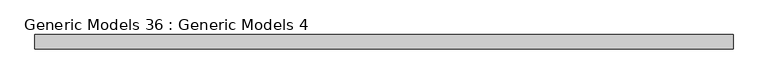
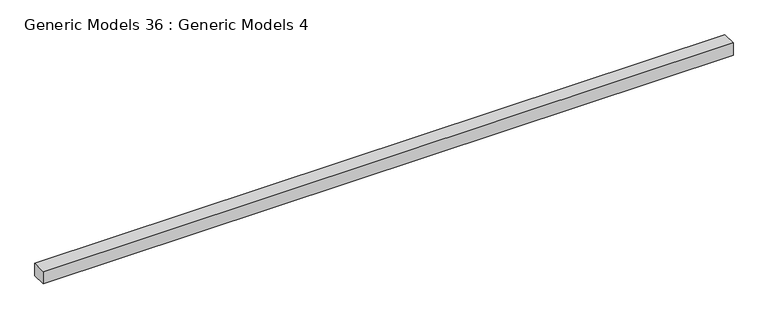
"""IFC4 building model written with IfcOpenShell, lengths in millimetres: proxy geometry, Generic Models 36 : Generic Models 4."""

from ifc_helpers import new_model, si_unit, frame, origin, place, context, project, spatial, polyline, outline, extrude, source, transform, mapped, element, save


def generic_models_36_generic_models_4_c2a80e1e(model_context):
    return source(origin(), model_context, "Body", "SweptSolid", [
        extrude(outline(polyline([(8409.0828684, 11880.2769662), (8409.0828684, 11499.2769662), (-10234.5171316, 11499.2769662), (-10234.5171316, 11880.2769662), (8409.0828684, 11880.2769662)])), frame((0.0, 0.0, 126402.846), z_axis=(0.0, 0.0, 1.0), x_axis=(1.0, 0.0, 0.0)), (0.0, 0.0, 1.0), 347.5929632),
    ])


if __name__ == "__main__":
    model = new_model("IFC4")
    model_context = context("Model", 3, world=origin())
    ifc_project = project(units=[si_unit("LENGTHUNIT", "METRE", prefix="MILLI")], contexts=[model_context])
    site = spatial("IfcSite", under=ifc_project)
    building = spatial("IfcBuilding", under=site)
    placement = place(None, origin())
    generic_models_36_generic_models_4_shape = generic_models_36_generic_models_4_c2a80e1e(model_context)
    element("IfcBuildingElementProxy", 1, Name="Generic Models 36 : Generic Models 4", ObjectType="Generic Models 36 : Generic Models 4", at=placement, inside=building, context=model_context, shape_type="MappedRepresentation", body=[
        mapped(generic_models_36_generic_models_4_shape, transform((0.0, 0.0, 0.0), x_axis=(1.0, 0.0, 0.0), y_axis=(0.0, 1.0, 0.0), z_axis=(0.0, 0.0, 1.0))),
    ])
    save(model, "model.ifc")

# Revit data of these elements
# Element 1 (IfcBuildingElementProxy, "Generic Models 36 : Generic Models 4")
#   Materials on its faces: "_BATT INSUL. (R-FACTOR = R38 MIN) OVER CLASS II VAPOR RETARDER(TOWARD INTERIOR)"
# Materials
#   "_BATT INSUL. (R-FACTOR = R38 MIN) OVER CLASS II VAPOR RETARDER(TOWARD INTERIOR)": class "Generic", colour RGB 227 210 251, transparency 0, Cost = 0
